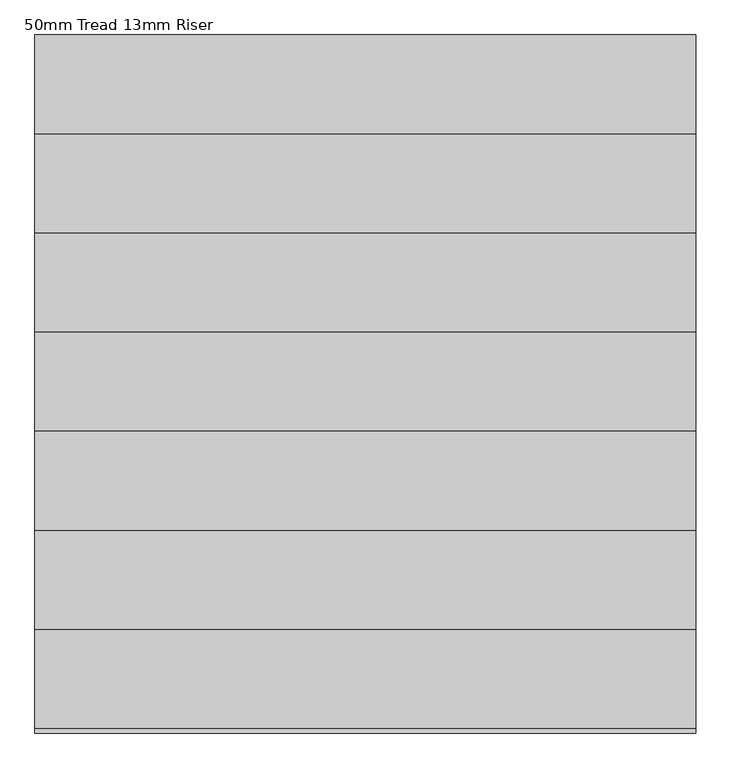
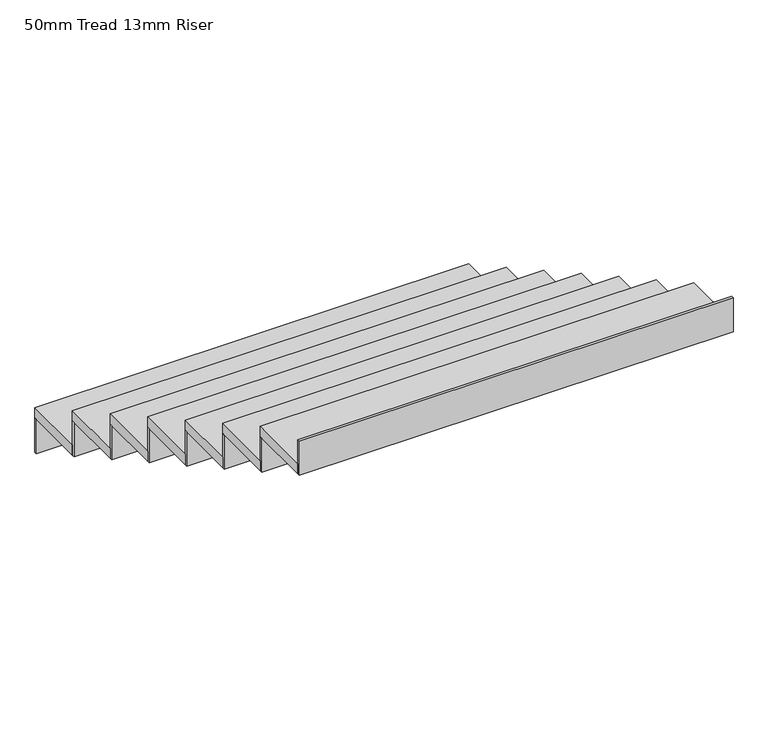
"""IFC4 building model written with IfcOpenShell, lengths in millimetres: stair flight geometry, 50mm Tread 13mm Riser."""

from ifc_helpers import new_model, si_unit, frame, origin, place, context, project, spatial, polyline, outline, extrude, source, transform, mapped, element, save


def stair_flight_50mm_tread_13mm_riser_821fa6e6(model_context):
    return source(origin(), model_context, "Body", "SweptSolid", [
        extrude(outline(polyline([(15000.0002442, 23517.4999999), (15000.0002442, 23529.9999999), (17000.0002442, 23529.9999999), (17000.0002442, 23517.4999999), (15000.0002442, 23517.4999999)])), frame((0.0, 0.0, 27783.3333333), z_axis=(0.0, 0.0, 1.0), x_axis=(1.0, 0.0, 0.0)), (0.0, 0.0, 1.0), 166.6666667),
        extrude(outline(polyline([(17000.0002442, 23229.9999999), (15000.0002442, 23229.9999999), (15000.0002442, 23529.9999999), (17000.0002442, 23529.9999999), (17000.0002442, 23229.9999999)])), frame((0.0, 0.0, 27950.0), z_axis=(0.0, 0.0, 1.0), x_axis=(1.0, 0.0, 0.0)), (0.0, 0.0, 1.0), 50.0),
        extrude(outline(polyline([(15000.0002442, 23217.4999999), (15000.0002442, 23229.9999999), (17000.0002442, 23229.9999999), (17000.0002442, 23217.4999999), (15000.0002442, 23217.4999999)])), frame((0.0, 0.0, 27950.0), z_axis=(0.0, 0.0, 1.0), x_axis=(1.0, 0.0, 0.0)), (0.0, 0.0, 1.0), 166.6666667),
        extrude(outline(polyline([(17000.0002442, 22929.9999999), (15000.0002442, 22929.9999999), (15000.0002442, 23229.9999999), (17000.0002442, 23229.9999999), (17000.0002442, 22929.9999999)])), frame((0.0, 0.0, 28116.6666667), z_axis=(0.0, 0.0, 1.0), x_axis=(1.0, 0.0, 0.0)), (0.0, 0.0, 1.0), 50.0),
        extrude(outline(polyline([(15000.0002442, 22917.4999999), (15000.0002442, 22929.9999999), (17000.0002442, 22929.9999999), (17000.0002442, 22917.4999999), (15000.0002442, 22917.4999999)])), frame((0.0, 0.0, 28116.6666667), z_axis=(0.0, 0.0, 1.0), x_axis=(1.0, 0.0, 0.0)), (0.0, 0.0, 1.0), 166.6666667),
        extrude(outline(polyline([(17000.0002442, 22629.9999999), (15000.0002442, 22629.9999999), (15000.0002442, 22929.9999999), (17000.0002442, 22929.9999999), (17000.0002442, 22629.9999999)])), frame((0.0, 0.0, 28283.3333333), z_axis=(0.0, 0.0, 1.0), x_axis=(1.0, 0.0, 0.0)), (0.0, 0.0, 1.0), 50.0),
        extrude(outline(polyline([(15000.0002442, 22617.4999999), (15000.0002442, 22629.9999999), (17000.0002442, 22629.9999999), (17000.0002442, 22617.4999999), (15000.0002442, 22617.4999999)])), frame((0.0, 0.0, 28283.3333333), z_axis=(0.0, 0.0, 1.0), x_axis=(1.0, 0.0, 0.0)), (0.0, 0.0, 1.0), 166.6666667),
        extrude(outline(polyline([(17000.0002442, 22329.9999999), (15000.0002442, 22329.9999999), (15000.0002442, 22629.9999999), (17000.0002442, 22629.9999999), (17000.0002442, 22329.9999999)])), frame((0.0, 0.0, 28450.0), z_axis=(0.0, 0.0, 1.0), x_axis=(1.0, 0.0, 0.0)), (0.0, 0.0, 1.0), 50.0),
        extrude(outline(polyline([(15000.0002442, 22317.4999999), (15000.0002442, 22329.9999999), (17000.0002442, 22329.9999999), (17000.0002442, 22317.4999999), (15000.0002442, 22317.4999999)])), frame((0.0, 0.0, 28450.0), z_axis=(0.0, 0.0, 1.0), x_axis=(1.0, 0.0, 0.0)), (0.0, 0.0, 1.0), 166.6666667),
        extrude(outline(polyline([(17000.0002442, 22029.9999999), (15000.0002442, 22029.9999999), (15000.0002442, 22329.9999999), (17000.0002442, 22329.9999999), (17000.0002442, 22029.9999999)])), frame((0.0, 0.0, 28616.6666667), z_axis=(0.0, 0.0, 1.0), x_axis=(1.0, 0.0, 0.0)), (0.0, 0.0, 1.0), 50.0),
        extrude(outline(polyline([(15000.0002442, 22017.4999999), (15000.0002442, 22029.9999999), (17000.0002442, 22029.9999999), (17000.0002442, 22017.4999999), (15000.0002442, 22017.4999999)])), frame((0.0, 0.0, 28616.6666667), z_axis=(0.0, 0.0, 1.0), x_axis=(1.0, 0.0, 0.0)), (0.0, 0.0, 1.0), 166.6666667),
        extrude(outline(polyline([(17000.0002442, 21729.9999999), (15000.0002442, 21729.9999999), (15000.0002442, 22029.9999999), (17000.0002442, 22029.9999999), (17000.0002442, 21729.9999999)])), frame((0.0, 0.0, 28783.3333333), z_axis=(0.0, 0.0, 1.0), x_axis=(1.0, 0.0, 0.0)), (0.0, 0.0, 1.0), 50.0),
        extrude(outline(polyline([(15000.0002442, 21717.4999999), (15000.0002442, 21729.9999999), (17000.0002442, 21729.9999999), (17000.0002442, 21717.4999999), (15000.0002442, 21717.4999999)])), frame((0.0, 0.0, 28783.3333333), z_axis=(0.0, 0.0, 1.0), x_axis=(1.0, 0.0, 0.0)), (0.0, 0.0, 1.0), 166.6666667),
        extrude(outline(polyline([(15000.0002442, 21417.4999999), (15000.0002442, 21429.9999999), (17000.0002442, 21429.9999999), (17000.0002442, 21417.4999999), (15000.0002442, 21417.4999999)])), frame((0.0, 0.0, 28950.0), z_axis=(0.0, 0.0, 1.0), x_axis=(1.0, 0.0, 0.0)), (0.0, 0.0, 1.0), 166.6666667),
        extrude(outline(polyline([(17000.0002442, 21429.9999999), (15000.0002442, 21429.9999999), (15000.0002442, 21729.9999999), (17000.0002442, 21729.9999999), (17000.0002442, 21429.9999999)])), frame((0.0, 0.0, 28950.0), z_axis=(0.0, 0.0, 1.0), x_axis=(1.0, 0.0, 0.0)), (0.0, 0.0, 1.0), 50.0),
    ])


if __name__ == "__main__":
    model = new_model("IFC4")
    model_context = context("Model", 3, world=origin())
    ifc_project = project(units=[si_unit("LENGTHUNIT", "METRE", prefix="MILLI")], contexts=[model_context])
    site = spatial("IfcSite", under=ifc_project)
    building = spatial("IfcBuilding", under=site)
    placement = place(None, origin())
    stair_flight_50mm_tread_13mm_riser_shape = stair_flight_50mm_tread_13mm_riser_821fa6e6(model_context)
    element("IfcStairFlight", 1, ObjectType="50mm Tread 13mm Riser", at=placement, inside=building, context=model_context, shape_type="MappedRepresentation", body=[
        mapped(stair_flight_50mm_tread_13mm_riser_shape, transform((0.0, 0.0, 0.0), x_axis=(1.0, 0.0, 0.0), y_axis=(0.0, 1.0, 0.0), z_axis=(0.0, 0.0, 1.0))),
    ])
    save(model, "model.ifc")
